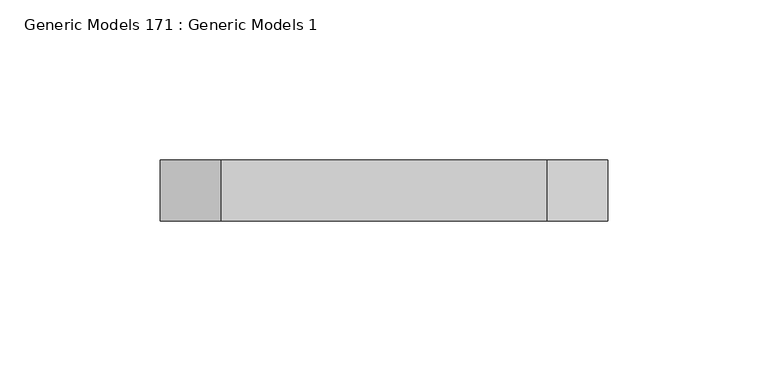
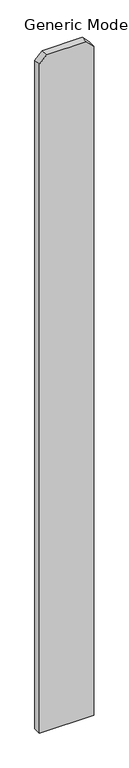
"""IFC4 building model written with IfcOpenShell, lengths in millimetres: proxy geometry, Generic Models 171 : Generic Models 1."""

from ifc_helpers import new_model, si_unit, frame, origin, place, context, project, spatial, polyline, outline, extrude, source, transform, mapped, element, save


def generic_models_171_generic_models_1_0cbeaef3(model_context):
    return source(origin(), model_context, "Body", "SweptSolid", [
        extrude(outline(polyline([(76.2, -248743.7875), (1885.95, -248743.7875), (1905.0, -248762.8375), (1905.0, -248864.4375), (1885.95, -248883.4875), (76.2, -248883.4875), (76.2, -248743.7875)])), frame((0.0, 547.6875, 0.0), z_axis=(0.0, 1.0, 0.0), x_axis=(0.0, 0.0, 1.0)), (0.0, 0.0, 1.0), 19.05),
    ])


if __name__ == "__main__":
    model = new_model("IFC4")
    model_context = context("Model", 3, world=origin())
    ifc_project = project(units=[si_unit("LENGTHUNIT", "METRE", prefix="MILLI")], contexts=[model_context])
    site = spatial("IfcSite", under=ifc_project)
    building = spatial("IfcBuilding", under=site)
    placement = place(None, origin())
    generic_models_171_generic_models_1_shape = generic_models_171_generic_models_1_0cbeaef3(model_context)
    element("IfcBuildingElementProxy", 1, Name="Generic Models 171 : Generic Models 1", ObjectType="Generic Models 171 : Generic Models 1", at=placement, inside=building, context=model_context, shape_type="MappedRepresentation", body=[
        mapped(generic_models_171_generic_models_1_shape, transform((0.0, 0.0, 0.0), x_axis=(1.0, 0.0, 0.0), y_axis=(0.0, 1.0, 0.0), z_axis=(0.0, 0.0, 1.0))),
    ])
    save(model, "model.ifc")

# Revit data of these elements
# Element 1 (IfcBuildingElementProxy, "Generic Models 171 : Generic Models 1")
#   Materials on its faces: "VERTICAL 1X6 CEDAR PLANKS W/ CLEAR WOOD SEALER"
# Materials
#   "VERTICAL 1X6 CEDAR PLANKS W/ CLEAR WOOD SEALER": class "Wood", colour RGB 234 198 147, transparency 0, Description = "Pinus Echinata", Cost = 0
